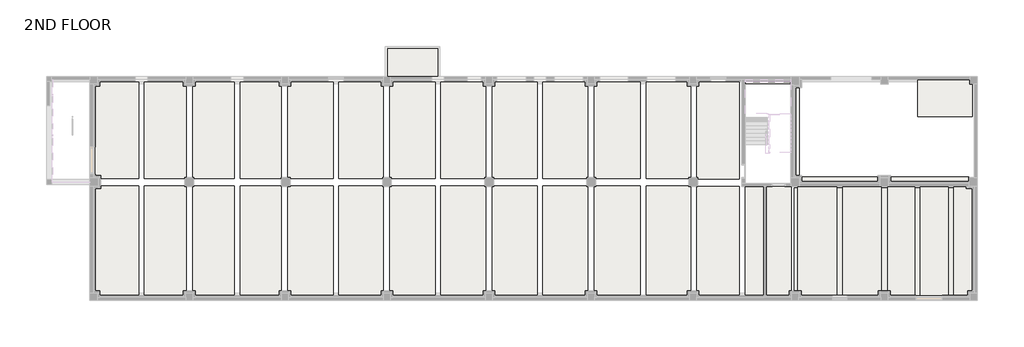
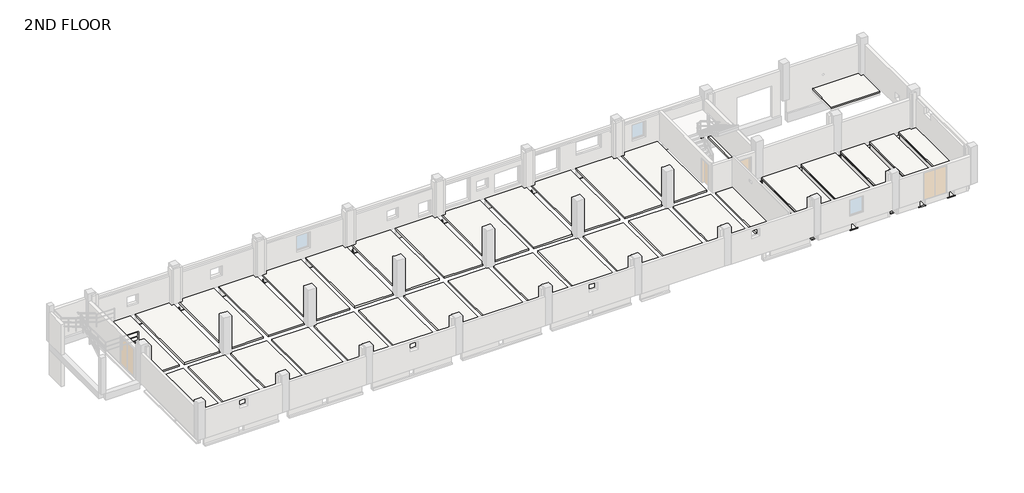
# One storey, part 4 of 7: 8 slabs, 2 coverings, 1 roof.
"""IFC4 building model written with IfcOpenShell, lengths in millimetres."""

from ifc_helpers import new_model, si_unit, frame, origin, place, context, project, spatial, polyline, outline, extrude, faceted_brep, element, save

model = new_model("IFC4")

# Units and contexts
model_context = context("Model", 3, world=origin())
ifc_project = project(units=[si_unit("LENGTHUNIT", "METRE", prefix="MILLI")], contexts=[model_context])

# Site, building, storey
site = spatial("IfcSite", under=ifc_project)
building = spatial("IfcBuilding", under=site)
storey = spatial("IfcBuildingStorey", under=building, Name="2ND FLOOR", Elevation=10600.0)

# Coverings
placement = place(None, origin())
element("IfcCovering", 1, ObjectType="H_CE_AR_B09_Souns Absorbing_100T_C7", at=placement, inside=storey, context=model_context, shape_type="SweptSolid", body=[
    extrude(outline(polyline([(58275.0, -8350.0), (58275.0, -16900.0), (55300.0, -16900.0), (55300.0, -16700.0), (55200.0, -16700.0), (55200.0, -8350.0), (58275.0, -8350.0)])), frame((0.0, 0.0, 10350.0), z_axis=(0.0, 0.0, 1.0), x_axis=(1.0, 0.0, 0.0)), (0.0, 0.0, 1.0), 100.0),
    extrude(outline(polyline([(58725.0, -8350.0), (61750.0, -8350.0), (61750.0, -16700.0), (61700.0, -16700.0), (61700.0, -16900.0), (58725.0, -16900.0), (58725.0, -8350.0)])), frame((0.0, 0.0, 10350.0), z_axis=(0.0, 0.0, 1.0), x_axis=(1.0, 0.0, 0.0)), (0.0, 0.0, 1.0), 100.0),
    extrude(outline(polyline([(64375.0, -8350.0), (64375.0, -16900.0), (62300.0, -16900.0), (62300.0, -16700.0), (62250.0, -16700.0), (62250.0, -8350.0), (64375.0, -8350.0)])), frame((0.0, 0.0, 10350.0), z_axis=(0.0, 0.0, 1.0), x_axis=(1.0, 0.0, 0.0)), (0.0, 0.0, 1.0), 100.0),
    extrude(outline(polyline([(67000.0, -8350.0), (67000.0, -16900.0), (64825.0, -16900.0), (64825.0, -8350.0), (67000.0, -8350.0)])), frame((0.0, 0.0, 10350.0), z_axis=(0.0, 0.0, 1.0), x_axis=(1.0, 0.0, 0.0)), (0.0, 0.0, 1.0), 100.0),
    extrude(outline(polyline([(68700.0, -16900.0), (67450.0, -16900.0), (67450.0, -8350.0), (68900.0, -8350.0), (68900.0, -16700.0), (68700.0, -16700.0), (68700.0, -16900.0)])), frame((0.0, 0.0, 10350.0), z_axis=(0.0, 0.0, 1.0), x_axis=(1.0, 0.0, 0.0)), (0.0, 0.0, 1.0), 100.0),
])
element("IfcCovering", 2, ObjectType="H_CE_AR_B09_Souns Absorbing_100T_C7", at=placement, inside=storey, context=model_context, shape_type="SweptSolid", body=[
    extrude(outline(polyline([(58175.0, -16886.0), (58175.0, -8469.0), (58825.0, -8469.0), (58825.0, -16886.0), (58175.0, -16886.0)])), frame((0.0, 0.0, 9700.0), z_axis=(0.0, 0.0, 1.0), x_axis=(1.0, 0.0, 0.0)), (0.0, 0.0, 1.0), 100.0),
    extrude(outline(polyline([(61650.0, -16536.0), (61650.0, -8469.0), (62350.0, -8469.0), (62350.0, -16536.0), (61650.0, -16536.0)])), frame((0.0, 0.0, 9700.0), z_axis=(0.0, 0.0, 1.0), x_axis=(1.0, 0.0, 0.0)), (0.0, 0.0, 1.0), 100.0),
    extrude(outline(polyline([(64275.0, -16886.0), (64275.0, -8469.0), (64925.0, -8469.0), (64925.0, -16886.0), (64275.0, -16886.0)])), frame((0.0, 0.0, 9700.0), z_axis=(0.0, 0.0, 1.0), x_axis=(1.0, 0.0, 0.0)), (0.0, 0.0, 1.0), 100.0),
    extrude(outline(polyline([(66900.0, -16886.0), (66900.0, -8469.0), (67550.0, -8469.0), (67550.0, -16886.0), (66900.0, -16886.0)])), frame((0.0, 0.0, 9700.0), z_axis=(0.0, 0.0, 1.0), x_axis=(1.0, 0.0, 0.0)), (0.0, 0.0, 1.0), 100.0),
    extrude(outline(polyline([(54937.0, -8469.0), (55300.0, -8469.0), (55300.0, -16536.0), (54937.0, -16536.0), (54937.0, -8469.0)])), frame((0.0, 0.0, 9700.0), z_axis=(0.0, 0.0, 1.0), x_axis=(1.0, 0.0, 0.0)), (0.0, 0.0, 1.0), 100.0),
])

# Roof
element("IfcRoof", 3, ObjectType="H_RF_AR_B06_RC Roof Finish_SkyPanel Roof_T160", at=placement, inside=storey, context=model_context, shape_type="SweptSolid", body=[
    extrude(outline(polyline([(23000.0, 2500.0), (27000.0, 2500.0), (27000.0, 300.0), (23000.0, 300.0), (23000.0, 2500.0)])), frame((0.0, 0.0, 9300.0), z_axis=(0.0, 0.0, 1.0), x_axis=(1.0, 0.0, 0.0)), (0.0, 0.0, 1.0), 170.0),
])

# Slabs
element("IfcSlab", 4, ObjectType="H_FL_AR_S17_RC Slab_T150_2S1", at=placement, inside=storey, context=model_context, shape_type="Brep", body=[
    faceted_brep([(3525.0, -100.0, 10450.0), (3525.0, -7700.0, 10450.0), (400.0, -7700.0, 10450.0), (399.4974747, -7700.0, 10450.0), (399.4974747, -7650.0, 10450.0), (100.0, -7650.0, 10450.0), (100.0, -300.0, 10450.0), (300.0, -300.0, 10450.0), (300.0, -100.0, 10450.0), (3525.0, -100.0, 10600.0), (300.0, -100.0, 10600.0), (300.0, -300.0, 10600.0), (100.0, -300.0, 10600.0), (100.0, -7650.0, 10600.0), (399.4974747, -7650.0, 10600.0), (399.4974747, -7700.0, 10600.0), (400.0, -7700.0, 10600.0), (3525.0, -7700.0, 10600.0)], [[[0, 1, 2, 3, 4, 5, 6, 7, 8]], [[9, 10, 11, 12, 13, 14, 15, 16, 17]], [[1, 0, 9, 17]], [[3, 2, 1, 17, 16, 15]], [[4, 3, 15, 14]], [[5, 4, 14, 13]], [[6, 5, 13, 12]], [[7, 6, 12, 11]], [[8, 7, 11, 10]], [[0, 8, 10, 9]]]),
    faceted_brep([(3975.0, -100.0, 10450.0), (7200.0, -100.0, 10450.0), (7200.0, -300.0, 10450.0), (7250.0, -300.0, 10450.0), (7250.0, -7650.0, 10450.0), (7150.0, -7650.0, 10450.0), (7150.0, -7700.0, 10450.0), (3975.0, -7700.0, 10450.0), (3975.0, -100.0, 10600.0), (3975.0, -7700.0, 10600.0), (7150.0, -7700.0, 10600.0), (7150.0, -7650.0, 10600.0), (7250.0, -7650.0, 10600.0), (7250.0, -300.0, 10600.0), (7200.0, -300.0, 10600.0), (7200.0, -100.0, 10600.0)], [[[0, 1, 2, 3, 4, 5, 6, 7]], [[8, 9, 10, 11, 12, 13, 14, 15]], [[1, 0, 8, 15]], [[2, 1, 15, 14]], [[3, 2, 14, 13]], [[4, 3, 13, 12]], [[5, 4, 12, 11]], [[6, 5, 11, 10]], [[7, 6, 10, 9]], [[0, 7, 9, 8]]]),
    faceted_brep([(3525.0, -16900.0, 10450.0), (300.0, -16900.0, 10450.0), (300.0, -16700.0, 10450.0), (100.0, -16700.0, 10450.0), (100.0, -8350.0, 10450.0), (399.4974747, -8350.0, 10450.0), (399.4974747, -8300.0, 10450.0), (400.0, -8300.0, 10450.0), (3525.0, -8300.0, 10450.0), (3525.0, -16900.0, 10600.0), (3525.0, -8300.0, 10600.0), (400.0, -8300.0, 10600.0), (399.4974747, -8300.0, 10600.0), (399.4974747, -8350.0, 10600.0), (100.0, -8350.0, 10600.0), (100.0, -16700.0, 10600.0), (300.0, -16700.0, 10600.0), (300.0, -16900.0, 10600.0)], [[[0, 1, 2, 3, 4, 5, 6, 7, 8]], [[9, 10, 11, 12, 13, 14, 15, 16, 17]], [[1, 0, 9, 17]], [[2, 1, 17, 16]], [[3, 2, 16, 15]], [[4, 3, 15, 14]], [[5, 4, 14, 13]], [[6, 5, 13, 12]], [[8, 7, 6, 12, 11, 10]], [[0, 8, 10, 9]]]),
    faceted_brep([(3975.0, -16900.0, 10450.0), (3975.0, -8300.0, 10450.0), (7150.0, -8300.0, 10450.0), (7150.0, -8350.0, 10450.0), (7250.0, -8350.0, 10450.0), (7250.0, -16700.0, 10450.0), (7200.0, -16700.0, 10450.0), (7200.0, -16900.0, 10450.0), (3975.0, -16900.0, 10600.0), (7200.0, -16900.0, 10600.0), (7200.0, -16700.0, 10600.0), (7250.0, -16700.0, 10600.0), (7250.0, -8350.0, 10600.0), (7150.0, -8350.0, 10600.0), (7150.0, -8300.0, 10600.0), (3975.0, -8300.0, 10600.0)], [[[0, 1, 2, 3, 4, 5, 6, 7]], [[8, 9, 10, 11, 12, 13, 14, 15]], [[1, 0, 8, 15]], [[2, 1, 15, 14]], [[3, 2, 14, 13]], [[4, 3, 13, 12]], [[5, 4, 12, 11]], [[6, 5, 11, 10]], [[7, 6, 10, 9]], [[0, 7, 9, 8]]]),
    faceted_brep([(11025.0, -100.0, 10450.0), (11025.0, -7700.0, 10450.0), (7850.0, -7700.0, 10450.0), (7850.0, -7650.0, 10450.0), (7750.0, -7650.0, 10450.0), (7750.0, -300.0, 10450.0), (7800.0, -300.0, 10450.0), (7800.0, -100.0, 10450.0), (11025.0, -100.0, 10600.0), (7800.0, -100.0, 10600.0), (7800.0, -300.0, 10600.0), (7750.0, -300.0, 10600.0), (7750.0, -7650.0, 10600.0), (7850.0, -7650.0, 10600.0), (7850.0, -7700.0, 10600.0), (11025.0, -7700.0, 10600.0)], [[[0, 1, 2, 3, 4, 5, 6, 7]], [[8, 9, 10, 11, 12, 13, 14, 15]], [[1, 0, 8, 15]], [[2, 1, 15, 14]], [[3, 2, 14, 13]], [[4, 3, 13, 12]], [[5, 4, 12, 11]], [[6, 5, 11, 10]], [[7, 6, 10, 9]], [[0, 7, 9, 8]]]),
    faceted_brep([(11025.0, -16900.0, 10450.0), (7800.0, -16900.0, 10450.0), (7800.0, -16700.0, 10450.0), (7750.0, -16700.0, 10450.0), (7750.0, -8350.0, 10450.0), (7850.0, -8350.0, 10450.0), (7850.0, -8300.0, 10450.0), (11025.0, -8300.0, 10450.0), (11025.0, -16900.0, 10600.0), (11025.0, -8300.0, 10600.0), (7850.0, -8300.0, 10600.0), (7850.0, -8350.0, 10600.0), (7750.0, -8350.0, 10600.0), (7750.0, -16700.0, 10600.0), (7800.0, -16700.0, 10600.0), (7800.0, -16900.0, 10600.0)], [[[0, 1, 2, 3, 4, 5, 6, 7]], [[8, 9, 10, 11, 12, 13, 14, 15]], [[1, 0, 8, 15]], [[2, 1, 15, 14]], [[3, 2, 14, 13]], [[4, 3, 13, 12]], [[5, 4, 12, 11]], [[6, 5, 11, 10]], [[7, 6, 10, 9]], [[0, 7, 9, 8]]]),
    faceted_brep([(14700.0, -100.0, 10450.0), (14700.0, -7700.0, 10450.0), (11475.0, -7700.0, 10450.0), (11475.0, -100.0, 10450.0), (14700.0, -100.0, 10600.0), (11475.0, -100.0, 10600.0), (11475.0, -7700.0, 10600.0), (14700.0, -7700.0, 10600.0), (14700.0, -7650.0, 10600.0), (14700.0, -300.0, 10600.0)], [[[0, 1, 2, 3]], [[4, 5, 6, 7, 8, 9]], [[1, 0, 4, 9, 8, 7]], [[2, 1, 7, 6]], [[3, 2, 6, 5]], [[0, 3, 5, 4]]]),
    faceted_brep([(11475.0, -8300.0, 10450.0), (14700.0, -8300.0, 10450.0), (14700.0, -16900.0, 10450.0), (11475.0, -16900.0, 10450.0), (11475.0, -8300.0, 10600.0), (11475.0, -16900.0, 10600.0), (14700.0, -16900.0, 10600.0), (14700.0, -16700.0, 10600.0), (14700.0, -8350.0, 10600.0), (14700.0, -8300.0, 10600.0)], [[[0, 1, 2, 3]], [[4, 5, 6, 7, 8, 9]], [[1, 0, 4, 9]], [[2, 1, 9, 8, 7, 6]], [[3, 2, 6, 5]], [[0, 3, 5, 4]]]),
    faceted_brep([(15300.0, -300.0, 10450.0), (15300.0, -100.0, 10450.0), (18775.0, -100.0, 10450.0), (18775.0, -7700.0, 10450.0), (15400.0000001, -7700.0, 10450.0), (15400.0000001, -7650.0, 10450.0), (15200.0, -7650.0, 10450.0), (15200.0, -300.0, 10450.0), (15300.0, -300.0, 10600.0), (15200.0, -300.0, 10600.0), (15200.0, -7650.0, 10600.0), (15400.0000001, -7650.0, 10600.0), (15400.0000001, -7700.0, 10600.0), (18775.0, -7700.0, 10600.0), (18775.0, -100.0, 10600.0), (15300.0, -100.0, 10600.0)], [[[0, 1, 2, 3, 4, 5, 6, 7]], [[8, 9, 10, 11, 12, 13, 14, 15]], [[1, 0, 8, 15]], [[2, 1, 15, 14]], [[3, 2, 14, 13]], [[4, 3, 13, 12]], [[5, 4, 12, 11]], [[6, 5, 11, 10]], [[7, 6, 10, 9]], [[0, 7, 9, 8]]]),
    faceted_brep([(15300.0, -16700.0, 10450.0), (15200.0, -16700.0, 10450.0), (15200.0, -8350.0, 10450.0), (15400.0000001, -8350.0, 10450.0), (15400.0000001, -8300.0, 10450.0), (18775.0, -8300.0, 10450.0), (18775.0, -16900.0, 10450.0), (15300.0, -16900.0, 10450.0), (15300.0, -16700.0, 10600.0), (15300.0, -16900.0, 10600.0), (18775.0, -16900.0, 10600.0), (18775.0, -8300.0, 10600.0), (15400.0000001, -8300.0, 10600.0), (15400.0000001, -8350.0, 10600.0), (15200.0, -8350.0, 10600.0), (15200.0, -16700.0, 10600.0)], [[[0, 1, 2, 3, 4, 5, 6, 7]], [[8, 9, 10, 11, 12, 13, 14, 15]], [[1, 0, 8, 15]], [[2, 1, 15, 14]], [[3, 2, 14, 13]], [[4, 3, 13, 12]], [[5, 4, 12, 11]], [[6, 5, 11, 10]], [[7, 6, 10, 9]], [[0, 7, 9, 8]]]),
    faceted_brep([(19225.0, -100.0, 10450.0), (22700.0, -100.0, 10450.0), (22700.0, -7650.0, 10450.0), (22650.0000003, -7650.0, 10450.0), (22650.0000003, -7700.0, 10450.0), (19225.0, -7700.0, 10450.0), (19225.0, -100.0, 10600.0), (19225.0, -7700.0, 10600.0), (22650.0000003, -7700.0, 10600.0), (22650.0000003, -7650.0, 10600.0), (22700.0, -7650.0, 10600.0), (22700.0, -300.0, 10600.0), (22700.0, -100.0, 10600.0)], [[[0, 1, 2, 3, 4, 5]], [[6, 7, 8, 9, 10, 11, 12]], [[1, 0, 6, 12]], [[2, 1, 12, 11, 10]], [[3, 2, 10, 9]], [[4, 3, 9, 8]], [[5, 4, 8, 7]], [[0, 5, 7, 6]]]),
    faceted_brep([(19225.0, -16900.0, 10450.0), (19225.0, -8300.0, 10450.0), (22650.0000003, -8300.0, 10450.0), (22650.0000003, -8350.0, 10450.0), (22700.0, -8350.0, 10450.0), (22700.0, -16900.0, 10450.0), (19225.0, -16900.0, 10600.0), (22700.0, -16900.0, 10600.0), (22700.0, -16700.0, 10600.0), (22700.0, -8350.0, 10600.0), (22650.0000003, -8350.0, 10600.0), (22650.0000003, -8300.0, 10600.0), (19225.0, -8300.0, 10600.0)], [[[0, 1, 2, 3, 4, 5]], [[6, 7, 8, 9, 10, 11, 12]], [[1, 0, 6, 12]], [[2, 1, 12, 11]], [[3, 2, 11, 10]], [[4, 3, 10, 9]], [[5, 4, 9, 8, 7]], [[0, 5, 7, 6]]]),
    faceted_brep([(23300.0, -100.0, 10450.0), (26775.0, -100.0, 10450.0), (26775.0, -7700.0, 10450.0), (23350.0000003, -7700.0, 10450.0), (23350.0000003, -7650.0, 10450.0), (23200.0, -7650.0, 10450.0), (23200.0, -300.0, 10450.0), (23300.0, -300.0, 10450.0), (23300.0, -100.0, 10600.0), (23300.0, -300.0, 10600.0), (23200.0, -300.0, 10600.0), (23200.0, -7650.0, 10600.0), (23350.0000003, -7650.0, 10600.0), (23350.0000003, -7700.0, 10600.0), (26775.0, -7700.0, 10600.0), (26775.0, -100.0, 10600.0)], [[[0, 1, 2, 3, 4, 5, 6, 7]], [[8, 9, 10, 11, 12, 13, 14, 15]], [[1, 0, 8, 15]], [[2, 1, 15, 14]], [[3, 2, 14, 13]], [[4, 3, 13, 12]], [[5, 4, 12, 11]], [[6, 5, 11, 10]], [[7, 6, 10, 9]], [[0, 7, 9, 8]]]),
    faceted_brep([(23300.0, -16900.0, 10450.0), (23300.0, -16700.0, 10450.0), (23200.0, -16700.0, 10450.0), (23200.0, -8350.0, 10450.0), (23350.0000003, -8350.0, 10450.0), (23350.0000003, -8300.0, 10450.0), (26775.0, -8300.0, 10450.0), (26775.0, -16900.0, 10450.0), (23300.0, -16900.0, 10600.0), (26775.0, -16900.0, 10600.0), (26775.0, -8300.0, 10600.0), (23350.0000003, -8300.0, 10600.0), (23350.0000003, -8350.0, 10600.0), (23200.0, -8350.0, 10600.0), (23200.0, -16700.0, 10600.0), (23300.0, -16700.0, 10600.0)], [[[0, 1, 2, 3, 4, 5, 6, 7]], [[8, 9, 10, 11, 12, 13, 14, 15]], [[1, 0, 8, 15]], [[2, 1, 15, 14]], [[3, 2, 14, 13]], [[4, 3, 13, 12]], [[5, 4, 12, 11]], [[6, 5, 11, 10]], [[7, 6, 10, 9]], [[0, 7, 9, 8]]]),
    faceted_brep([(30700.0, -100.0, 10450.0), (30700.0, -300.0, 10450.0), (30750.0000002, -300.0, 10450.0), (30750.0000002, -7650.0, 10450.0), (30649.9999997, -7650.0, 10450.0), (30649.9999997, -7700.0, 10450.0), (27225.0, -7700.0, 10450.0), (27225.0, -100.0, 10450.0), (30700.0, -100.0, 10600.0), (27225.0, -100.0, 10600.0), (27225.0, -7700.0, 10600.0), (30649.9999997, -7700.0, 10600.0), (30649.9999997, -7650.0, 10600.0), (30750.0000002, -7650.0, 10600.0), (30750.0000002, -300.0, 10600.0), (30700.0, -300.0, 10600.0)], [[[0, 1, 2, 3, 4, 5, 6, 7]], [[8, 9, 10, 11, 12, 13, 14, 15]], [[1, 0, 8, 15]], [[2, 1, 15, 14]], [[3, 2, 14, 13]], [[4, 3, 13, 12]], [[5, 4, 12, 11]], [[6, 5, 11, 10]], [[7, 6, 10, 9]], [[0, 7, 9, 8]]]),
    faceted_brep([(30700.0, -16900.0, 10450.0), (27225.0, -16900.0, 10450.0), (27225.0, -8300.0, 10450.0), (30649.9999997, -8300.0, 10450.0), (30649.9999997, -8350.0, 10450.0), (30750.0000002, -8350.0, 10450.0), (30750.0000002, -16700.0, 10450.0), (30700.0, -16700.0, 10450.0), (30700.0, -16900.0, 10600.0), (30700.0, -16700.0, 10600.0), (30750.0000002, -16700.0, 10600.0), (30750.0000002, -8350.0, 10600.0), (30649.9999997, -8350.0, 10600.0), (30649.9999997, -8300.0, 10600.0), (27225.0, -8300.0, 10600.0), (27225.0, -16900.0, 10600.0)], [[[0, 1, 2, 3, 4, 5, 6, 7]], [[8, 9, 10, 11, 12, 13, 14, 15]], [[1, 0, 8, 15]], [[2, 1, 15, 14]], [[3, 2, 14, 13]], [[4, 3, 13, 12]], [[5, 4, 12, 11]], [[6, 5, 11, 10]], [[7, 6, 10, 9]], [[0, 7, 9, 8]]]),
    faceted_brep([(31300.0, -100.0, 10450.0), (34775.0, -100.0, 10450.0), (34775.0, -7700.0, 10450.0), (31350.0000003, -7700.0, 10450.0), (31350.0000003, -7650.0, 10450.0), (31249.9999998, -7650.0, 10450.0), (31249.9999998, -300.0, 10450.0), (31300.0, -300.0, 10450.0), (31300.0, -100.0, 10600.0), (31300.0, -300.0, 10600.0), (31249.9999998, -300.0, 10600.0), (31249.9999998, -7650.0, 10600.0), (31350.0000003, -7650.0, 10600.0), (31350.0000003, -7700.0, 10600.0), (34775.0, -7700.0, 10600.0), (34775.0, -100.0, 10600.0)], [[[0, 1, 2, 3, 4, 5, 6, 7]], [[8, 9, 10, 11, 12, 13, 14, 15]], [[1, 0, 8, 15]], [[2, 1, 15, 14]], [[3, 2, 14, 13]], [[4, 3, 13, 12]], [[5, 4, 12, 11]], [[6, 5, 11, 10]], [[7, 6, 10, 9]], [[0, 7, 9, 8]]]),
    faceted_brep([(31300.0, -16900.0, 10450.0), (31300.0, -16700.0, 10450.0), (31249.9999998, -16700.0, 10450.0), (31249.9999998, -8350.0, 10450.0), (31350.0000003, -8350.0, 10450.0), (31350.0000003, -8300.0, 10450.0), (34775.0, -8300.0, 10450.0), (34775.0, -16900.0, 10450.0), (31300.0, -16900.0, 10600.0), (34775.0, -16900.0, 10600.0), (34775.0, -8300.0, 10600.0), (31350.0000003, -8300.0, 10600.0), (31350.0000003, -8350.0, 10600.0), (31249.9999998, -8350.0, 10600.0), (31249.9999998, -16700.0, 10600.0), (31300.0, -16700.0, 10600.0)], [[[0, 1, 2, 3, 4, 5, 6, 7]], [[8, 9, 10, 11, 12, 13, 14, 15]], [[1, 0, 8, 15]], [[2, 1, 15, 14]], [[3, 2, 14, 13]], [[4, 3, 13, 12]], [[5, 4, 12, 11]], [[6, 5, 11, 10]], [[7, 6, 10, 9]], [[0, 7, 9, 8]]]),
    faceted_brep([(38700.0, -100.0, 10450.0), (38700.0, -300.0, 10450.0), (38750.0000002, -300.0, 10450.0), (38750.0000002, -7650.0, 10450.0), (38649.9999997, -7650.0, 10450.0), (38649.9999997, -7700.0, 10450.0), (35225.0, -7700.0, 10450.0), (35225.0, -100.0, 10450.0), (38700.0, -100.0, 10600.0), (35225.0, -100.0, 10600.0), (35225.0, -7700.0, 10600.0), (38649.9999997, -7700.0, 10600.0), (38649.9999997, -7650.0, 10600.0), (38750.0000002, -7650.0, 10600.0), (38750.0000002, -300.0, 10600.0), (38700.0, -300.0, 10600.0)], [[[0, 1, 2, 3, 4, 5, 6, 7]], [[8, 9, 10, 11, 12, 13, 14, 15]], [[1, 0, 8, 15]], [[2, 1, 15, 14]], [[3, 2, 14, 13]], [[4, 3, 13, 12]], [[5, 4, 12, 11]], [[6, 5, 11, 10]], [[7, 6, 10, 9]], [[0, 7, 9, 8]]]),
    faceted_brep([(38700.0, -16900.0, 10450.0), (35225.0, -16900.0, 10450.0), (35225.0, -8300.0, 10450.0), (38649.9999997, -8300.0, 10450.0), (38649.9999997, -8350.0, 10450.0), (38750.0000002, -8350.0, 10450.0), (38750.0000002, -16700.0, 10450.0), (38700.0, -16700.0, 10450.0), (38700.0, -16900.0, 10600.0), (38700.0, -16700.0, 10600.0), (38750.0000002, -16700.0, 10600.0), (38750.0000002, -8350.0, 10600.0), (38649.9999997, -8350.0, 10600.0), (38649.9999997, -8300.0, 10600.0), (35225.0, -8300.0, 10600.0), (35225.0, -16900.0, 10600.0)], [[[0, 1, 2, 3, 4, 5, 6, 7]], [[8, 9, 10, 11, 12, 13, 14, 15]], [[1, 0, 8, 15]], [[2, 1, 15, 14]], [[3, 2, 14, 13]], [[4, 3, 13, 12]], [[5, 4, 12, 11]], [[6, 5, 11, 10]], [[7, 6, 10, 9]], [[0, 7, 9, 8]]]),
    faceted_brep([(39300.0, -100.0, 10450.0), (42875.0, -100.0, 10450.0), (42875.0, -7700.0, 10450.0), (39350.0000003, -7700.0, 10450.0), (39350.0000003, -7650.0, 10450.0), (39249.9999998, -7650.0, 10450.0), (39249.9999998, -300.0, 10450.0), (39300.0, -300.0, 10450.0), (39300.0, -100.0, 10600.0), (39300.0, -300.0, 10600.0), (39249.9999998, -300.0, 10600.0), (39249.9999998, -7650.0, 10600.0), (39350.0000003, -7650.0, 10600.0), (39350.0000003, -7700.0, 10600.0), (42875.0, -7700.0, 10600.0), (42875.0, -100.0, 10600.0)], [[[0, 1, 2, 3, 4, 5, 6, 7]], [[8, 9, 10, 11, 12, 13, 14, 15]], [[1, 0, 8, 15]], [[2, 1, 15, 14]], [[3, 2, 14, 13]], [[4, 3, 13, 12]], [[5, 4, 12, 11]], [[6, 5, 11, 10]], [[7, 6, 10, 9]], [[0, 7, 9, 8]]]),
    faceted_brep([(39300.0, -16900.0, 10450.0), (39300.0, -16700.0, 10450.0), (39249.9999998, -16700.0, 10450.0), (39249.9999998, -8350.0, 10450.0), (39350.0000003, -8350.0, 10450.0), (39350.0000003, -8300.0, 10450.0), (42875.0, -8300.0, 10450.0), (42875.0, -16900.0, 10450.0), (39300.0, -16900.0, 10600.0), (42875.0, -16900.0, 10600.0), (42875.0, -8300.0, 10600.0), (39350.0000003, -8300.0, 10600.0), (39350.0000003, -8350.0, 10600.0), (39249.9999998, -8350.0, 10600.0), (39249.9999998, -16700.0, 10600.0), (39300.0, -16700.0, 10600.0)], [[[0, 1, 2, 3, 4, 5, 6, 7]], [[8, 9, 10, 11, 12, 13, 14, 15]], [[1, 0, 8, 15]], [[2, 1, 15, 14]], [[3, 2, 14, 13]], [[4, 3, 13, 12]], [[5, 4, 12, 11]], [[6, 5, 11, 10]], [[7, 6, 10, 9]], [[0, 7, 9, 8]]]),
    faceted_brep([(46700.0, -100.0, 10450.0), (46700.0, -300.0, 10450.0), (46800.0, -300.0, 10450.0), (46800.0, -7650.0, 10450.0), (46649.9999999, -7650.0, 10450.0), (46649.9999999, -7700.0, 10450.0), (43325.0, -7700.0, 10450.0), (43325.0, -100.0, 10450.0), (46700.0, -100.0, 10600.0), (43325.0, -100.0, 10600.0), (43325.0, -7700.0, 10600.0), (46649.9999999, -7700.0, 10600.0), (46649.9999999, -7650.0, 10600.0), (46800.0, -7650.0, 10600.0), (46800.0, -300.0, 10600.0), (46700.0, -300.0, 10600.0)], [[[0, 1, 2, 3, 4, 5, 6, 7]], [[8, 9, 10, 11, 12, 13, 14, 15]], [[1, 0, 8, 15]], [[2, 1, 15, 14]], [[3, 2, 14, 13]], [[4, 3, 13, 12]], [[5, 4, 12, 11]], [[6, 5, 11, 10]], [[7, 6, 10, 9]], [[0, 7, 9, 8]]]),
    faceted_brep([(46700.0, -16900.0, 10450.0), (43325.0, -16900.0, 10450.0), (43325.0, -8300.0, 10450.0), (46649.9999999, -8300.0, 10450.0), (46649.9999999, -8350.0, 10450.0), (46800.0, -8350.0, 10450.0), (46800.0, -16700.0, 10450.0), (46700.0, -16700.0, 10450.0), (46700.0, -16900.0, 10600.0), (46700.0, -16700.0, 10600.0), (46800.0, -16700.0, 10600.0), (46800.0, -8350.0, 10600.0), (46649.9999999, -8350.0, 10600.0), (46649.9999999, -8300.0, 10600.0), (43325.0, -8300.0, 10600.0), (43325.0, -16900.0, 10600.0)], [[[0, 1, 2, 3, 4, 5, 6, 7]], [[8, 9, 10, 11, 12, 13, 14, 15]], [[1, 0, 8, 15]], [[2, 1, 15, 14]], [[3, 2, 14, 13]], [[4, 3, 13, 12]], [[5, 4, 12, 11]], [[6, 5, 11, 10]], [[7, 6, 10, 9]], [[0, 7, 9, 8]]]),
    faceted_brep([(50625.0, -8350.0, 10450.0), (50625.0, -16900.0, 10450.0), (47300.0, -16900.0, 10450.0), (47300.0, -8350.0, 10450.0), (50625.0, -8350.0, 10600.0), (47350.0, -8350.0, 10600.0), (47300.0, -8350.0, 10600.0), (47300.0, -16700.0, 10600.0), (47300.0, -16900.0, 10600.0), (50625.0, -16900.0, 10600.0)], [[[0, 1, 2, 3]], [[4, 5, 6, 7, 8, 9]], [[1, 0, 4, 9]], [[2, 1, 9, 8]], [[3, 2, 8, 7, 6]], [[0, 3, 6, 5, 4]]]),
    faceted_brep([(50625.0, -100.0, 10450.0), (50625.0, -7750.0, 10450.0), (47349.9999999, -7750.0, 10450.0), (47349.9999999, -7650.0, 10450.0), (47300.0, -7650.0, 10450.0), (47300.0, -100.0, 10450.0), (50625.0, -100.0, 10600.0), (47300.0, -100.0, 10600.0), (47300.0, -300.0, 10600.0), (47300.0, -7650.0, 10600.0), (47349.9999999, -7650.0, 10600.0), (47349.9999999, -7750.0, 10600.0), (50625.0, -7750.0, 10600.0)], [[[0, 1, 2, 3, 4, 5]], [[6, 7, 8, 9, 10, 11, 12]], [[1, 0, 6, 12]], [[2, 1, 12, 11]], [[3, 2, 11, 10]], [[4, 3, 10, 9]], [[5, 4, 9, 8, 7]], [[0, 5, 7, 6]]]),
    faceted_brep([(54700.0, -8350.0, 10450.0), (54700.0, -16900.0, 10450.0), (51075.0, -16900.0, 10450.0), (51075.0, -8350.0, 10450.0), (54700.0, -8350.0, 10600.0), (54650.0, -8350.0, 10600.0), (51075.0, -8350.0, 10600.0), (51075.0, -16900.0, 10600.0), (54700.0, -16900.0, 10600.0), (54700.0, -16700.0, 10600.0)], [[[0, 1, 2, 3]], [[4, 5, 6, 7, 8, 9]], [[1, 0, 4, 9, 8]], [[2, 1, 8, 7]], [[3, 2, 7, 6]], [[0, 3, 6, 5, 4]]]),
    faceted_brep([(58275.0, -8350.0, 10450.0), (58275.0, -16900.0, 10450.0), (55300.0, -16900.0, 10450.0), (55300.0, -16700.0, 10450.0), (55200.0, -16700.0, 10450.0), (55200.0, -8350.0, 10450.0), (58275.0, -8350.0, 10600.0), (55350.0, -8350.0, 10600.0), (55200.0, -8350.0, 10600.0), (55200.0, -16700.0, 10600.0), (55300.0, -16700.0, 10600.0), (55300.0, -16900.0, 10600.0), (58275.0, -16900.0, 10600.0)], [[[0, 1, 2, 3, 4, 5]], [[6, 7, 8, 9, 10, 11, 12]], [[1, 0, 6, 12]], [[2, 1, 12, 11]], [[3, 2, 11, 10]], [[4, 3, 10, 9]], [[5, 4, 9, 8]], [[0, 5, 8, 7, 6]]]),
    faceted_brep([(58725.0, -8350.0, 10450.0), (61750.0, -8350.0, 10450.0), (61750.0, -16700.0, 10450.0), (61700.0, -16700.0, 10450.0), (61700.0, -16900.0, 10450.0), (58725.0, -16900.0, 10450.0), (58725.0, -8350.0, 10600.0), (58725.0, -16900.0, 10600.0), (61700.0, -16900.0, 10600.0), (61700.0, -16700.0, 10600.0), (61750.0, -16700.0, 10600.0), (61750.0, -8350.0, 10600.0), (61650.0, -8350.0, 10600.0)], [[[0, 1, 2, 3, 4, 5]], [[6, 7, 8, 9, 10, 11, 12]], [[1, 0, 6, 12, 11]], [[2, 1, 11, 10]], [[3, 2, 10, 9]], [[4, 3, 9, 8]], [[5, 4, 8, 7]], [[0, 5, 7, 6]]]),
    faceted_brep([(64375.0, -8350.0, 10450.0), (64375.0, -16900.0, 10450.0), (62300.0, -16900.0, 10450.0), (62300.0, -16700.0, 10450.0), (62250.0, -16700.0, 10450.0), (62250.0, -8350.0, 10450.0), (64375.0, -8350.0, 10600.0), (62350.0, -8350.0, 10600.0), (62250.0, -8350.0, 10600.0), (62250.0, -16700.0, 10600.0), (62300.0, -16700.0, 10600.0), (62300.0, -16900.0, 10600.0), (64375.0, -16900.0, 10600.0)], [[[0, 1, 2, 3, 4, 5]], [[6, 7, 8, 9, 10, 11, 12]], [[1, 0, 6, 12]], [[2, 1, 12, 11]], [[3, 2, 11, 10]], [[4, 3, 10, 9]], [[5, 4, 9, 8]], [[0, 5, 8, 7, 6]]]),
    faceted_brep([(67000.0, -8350.0, 10450.0), (67000.0, -16900.0, 10450.0), (64825.0, -16900.0, 10450.0), (64825.0, -8350.0, 10450.0), (67000.0, -8350.0, 10600.0), (64825.0, -8350.0, 10600.0), (64825.0, -16900.0, 10600.0), (67000.0, -16900.0, 10600.0)], [[[0, 1, 2, 3]], [[4, 5, 6, 7]], [[1, 0, 4, 7]], [[2, 1, 7, 6]], [[3, 2, 6, 5]], [[0, 3, 5, 4]]]),
    faceted_brep([(68700.0, -16900.0, 10450.0), (67450.0, -16900.0, 10450.0), (67450.0, -8350.0, 10450.0), (68900.0, -8350.0, 10450.0), (68900.0, -16700.0, 10450.0), (68700.0, -16700.0, 10450.0), (68700.0, -16900.0, 10600.0), (68700.0, -16700.0, 10600.0), (68900.0, -16700.0, 10600.0), (68900.0, -8350.0, 10600.0), (68600.0, -8350.0, 10600.0), (67450.0, -8350.0, 10600.0), (67450.0, -16900.0, 10600.0)], [[[0, 1, 2, 3, 4, 5]], [[6, 7, 8, 9, 10, 11, 12]], [[1, 0, 6, 12]], [[2, 1, 12, 11]], [[3, 2, 11, 10, 9]], [[4, 3, 9, 8]], [[5, 4, 8, 7]], [[0, 5, 7, 6]]]),
])
element("IfcSlab", 5, ObjectType="H_FL_AR_S17_RC Slab_T150_2S2", at=placement, inside=storey, context=model_context, shape_type="SweptSolid", body=[
    extrude(outline(polyline([(68900.0, -2850.0), (64600.0, -2850.0), (64600.0, 50.0), (68700.0, 50.0), (68700.0, -300.0), (68900.0, -300.0), (68900.0, -2850.0)])), frame((0.0, 0.0, 10450.0), z_axis=(0.0, 0.0, 1.0), x_axis=(1.0, 0.0, 0.0)), (0.0, 0.0, 1.0), 150.0),
])
element("IfcSlab", 6, ObjectType="H_FL_AR_S17_RC Slab_T150_2CS1", at=placement, inside=storey, context=model_context, shape_type="SweptSolid", body=[
    extrude(outline(polyline([(26850.0, 2350.0), (26850.0, 300.0), (23150.0, 300.0), (23150.0, 2350.0), (26850.0, 2350.0)])), frame((0.0, 0.0, 9150.0), z_axis=(0.0, 0.0, 1.0), x_axis=(1.0, 0.0, 0.0)), (0.0, 0.0, 1.0), 150.0),
])
element("IfcSlab", 7, ObjectType="H_FL_AR_B07l_2L Gypsum_Insulationl_T154", at=placement, inside=storey, context=model_context, shape_type="Brep", body=[
    faceted_brep([(54910.0, -7486.0, 10600.0), (54910.0, -564.0, 10600.0), (55160.0, -564.0, 10600.0), (55160.0, -7486.0, 10600.0), (55314.0, -564.0, 10754.0), (55064.0, -564.0, 10754.0), (54910.0, -564.0, 10754.0), (54910.0, -7486.0, 10754.0), (55064.0, -7486.0, 10754.0), (55314.0, -7486.0, 10754.0), (55314.0, -564.0, 10735.0), (55160.0, -564.0, 10735.0), (55314.0, -7486.0, 10735.0), (54910.0, -7486.0, 10735.0), (55160.0, -7486.0, 10735.0)], [[[0, 1, 2, 3]], [[4, 5, 6, 7, 8, 9]], [[6, 5, 4, 10, 11, 2, 1]], [[4, 9, 12, 10]], [[9, 8, 7, 13, 0, 3, 14, 12]], [[1, 0, 13, 7, 6]], [[11, 14, 3, 2]], [[14, 11, 10, 12]]]),
    faceted_brep([(61486.0, -8090.0, 10600.0), (55514.0, -8090.0, 10600.0), (55514.0, -7740.0, 10600.0), (61486.0, -7740.0, 10600.0), (61486.0, -8090.0, 10754.0), (61486.0, -7936.0, 10754.0), (61486.0, -7586.0, 10754.0), (55514.0, -7586.0, 10754.0), (55514.0, -7936.0, 10754.0), (55514.0, -8090.0, 10754.0), (61486.0, -8090.0, 10735.0), (61486.0, -7740.0, 10735.0), (61486.0, -7586.0, 10735.0), (55514.0, -8090.0, 10735.0), (55514.0, -7586.0, 10735.0), (55514.0, -7740.0, 10735.0)], [[[0, 1, 2, 3]], [[4, 5, 6, 7, 8, 9]], [[6, 5, 4, 10, 0, 3, 11, 12]], [[1, 0, 10, 4, 9, 13]], [[9, 8, 7, 14, 15, 2, 1, 13]], [[7, 6, 12, 14]], [[15, 11, 3, 2]], [[11, 15, 14, 12]]]),
    faceted_brep([(68600.0, -8090.0, 10600.0), (62514.0, -8090.0, 10600.0), (62514.0, -7740.0, 10600.0), (68600.0, -7740.0, 10600.0), (68600.0, -8090.0, 10754.0), (68600.0, -7936.0, 10754.0), (68600.0, -7586.0, 10754.0), (62514.0, -7586.0, 10754.0), (62514.0, -7936.0, 10754.0), (62514.0, -8090.0, 10754.0), (68600.0, -7740.0, 10735.0), (68600.0, -7586.0, 10735.0), (62514.0, -7586.0, 10735.0), (62514.0, -7740.0, 10735.0)], [[[0, 1, 2, 3]], [[4, 5, 6, 7, 8, 9]], [[6, 5, 4, 0, 3, 10, 11]], [[1, 0, 4, 9]], [[9, 8, 7, 12, 13, 2, 1]], [[7, 6, 11, 12]], [[13, 10, 3, 2]], [[10, 13, 12, 11]]]),
])
element("IfcSlab", 8, ObjectType="H_WA_AR_B02_Int Wall_2L Gypsum_Insulationl_T154(Mirror)", at=placement, inside=storey, context=model_context, shape_type="Brep", body=[
    faceted_brep([(54910.0, -564.0, 9646.0), (55064.0, -564.0, 9646.0), (55314.0, -564.0, 9646.0), (55314.0, -7486.0, 9646.0), (55064.0, -7486.0, 9646.0), (54910.0, -7486.0, 9646.0), (54910.0, -564.0, 9800.0), (54910.0, -7486.0, 9800.0), (55160.0, -7486.0, 9800.0), (55160.0, -564.0, 9800.0), (55160.0, -564.0, 9665.0), (55314.0, -564.0, 9665.0), (55314.0, -7486.0, 9665.0), (55160.0, -7486.0, 9665.0), (54910.0, -7486.0, 9665.0)], [[[0, 1, 2, 3, 4, 5]], [[6, 7, 8, 9]], [[2, 1, 0, 6, 9, 10, 11]], [[3, 2, 11, 12]], [[5, 4, 3, 12, 13, 8, 7, 14]], [[0, 5, 14, 7, 6]], [[13, 10, 9, 8]], [[10, 13, 12, 11]]]),
    faceted_brep([(61486.0, -7586.0, 9646.0), (61486.0, -7936.0, 9646.0), (61486.0, -8090.0, 9646.0), (55514.0, -8090.0, 9646.0), (55514.0, -7936.0, 9646.0), (55514.0, -7586.0, 9646.0), (55514.0, -8090.0, 9800.0), (61486.0, -8090.0, 9800.0), (61486.0, -7740.0, 9800.0), (55514.0, -7740.0, 9800.0), (61486.0, -7586.0, 9665.0), (61486.0, -7740.0, 9665.0), (61486.0, -8090.0, 9665.0), (55514.0, -8090.0, 9665.0), (55514.0, -7740.0, 9665.0), (55514.0, -7586.0, 9665.0)], [[[0, 1, 2, 3, 4, 5]], [[6, 7, 8, 9]], [[2, 1, 0, 10, 11, 8, 7, 12]], [[3, 2, 12, 7, 6, 13]], [[5, 4, 3, 13, 6, 9, 14, 15]], [[0, 5, 15, 10]], [[11, 14, 9, 8]], [[14, 11, 10, 15]]]),
    faceted_brep([(68600.0, -7586.0, 9646.0), (68600.0, -7936.0, 9646.0), (68600.0, -8090.0, 9646.0), (62514.0, -8090.0, 9646.0), (62514.0, -7936.0, 9646.0), (62514.0, -7586.0, 9646.0), (62514.0, -8090.0, 9800.0), (68600.0, -8090.0, 9800.0), (68600.0, -7740.0, 9800.0), (62514.0, -7740.0, 9800.0), (68600.0, -7586.0, 9665.0), (68600.0, -7740.0, 9665.0), (62514.0, -7740.0, 9665.0), (62514.0, -7586.0, 9665.0)], [[[0, 1, 2, 3, 4, 5]], [[6, 7, 8, 9]], [[2, 1, 0, 10, 11, 8, 7]], [[3, 2, 7, 6]], [[5, 4, 3, 6, 9, 12, 13]], [[0, 5, 13, 10]], [[11, 12, 9, 8]], [[12, 11, 10, 13]]]),
])
element("IfcSlab", 9, ObjectType="H_WA_AR_B02_Int Wall_2L Gypsum_Insulationl_T154(Mirror)", at=placement, inside=storey, context=model_context, shape_type="Brep", body=[
    faceted_brep([(54650.0, -264.0, 9636.0), (51074.7487373, -264.0, 9636.0), (51074.7487373, 40.0, 9636.0), (51075.0, 40.0, 9636.0), (54650.0, 40.0, 9636.0), (54650.0, -114.0, 9636.0), (54650.0, 40.0, 9790.0), (51074.7487373, 40.0, 9790.0), (51074.7487373, -110.0, 9790.0), (54650.0, -110.0, 9790.0), (54650.0, -264.0, 9655.0), (51074.7487373, -264.0, 9655.0), (51074.7487373, -110.0, 9655.0), (54650.0, -110.0, 9655.0)], [[[0, 1, 2, 3, 4, 5]], [[6, 7, 8, 9]], [[1, 0, 10, 11]], [[2, 1, 11, 12, 8, 7]], [[4, 3, 2, 7, 6]], [[0, 5, 4, 6, 9, 13, 10]], [[12, 13, 9, 8]], [[13, 12, 11, 10]]]),
])
element("IfcSlab", 10, ObjectType="H_FL_AR_B07l_2L Gypsum_Insulationl_T154", at=placement, inside=storey, context=model_context, shape_type="Brep", body=[
    faceted_brep([(51074.7487373, 40.0, 10610.0), (54650.0, 40.0, 10610.0), (54650.0, -110.0, 10610.0), (51074.7487373, -110.0, 10610.0), (51074.7487373, -264.0, 10764.0), (54650.0, -264.0, 10764.0), (54650.0, -114.0, 10764.0), (54650.0, 40.0, 10764.0), (51074.7487373, 40.0, 10764.0), (51074.7487373, -114.0, 10764.0), (51074.7487373, -264.0, 10735.0), (54650.0, -264.0, 10735.0), (51074.7487373, -110.0, 10735.0), (54650.0, -110.0, 10735.0)], [[[0, 1, 2, 3]], [[4, 5, 6, 7, 8, 9]], [[5, 4, 10, 11]], [[4, 9, 8, 0, 3, 12, 10]], [[1, 0, 8, 7]], [[7, 6, 5, 11, 13, 2, 1]], [[13, 12, 3, 2]], [[12, 13, 11, 10]]]),
])
element("IfcSlab", 11, ObjectType="H_WA_AR_B02_Int Wall_2L Gypsum_Insulationl_T154(Mirror)", at=placement, inside=storey, context=model_context, shape_type="Brep", body=[
    faceted_brep([(2201.0, -264.0, 9636.0), (464.0, -264.0, 9636.0), (464.0, -114.0, 9636.0), (2201.0, -114.0, 9636.0), (464.0, -264.0, 9655.0), (464.0, -114.0, 9655.0), (2201.0, -264.0, 9655.0), (2201.0, -114.0, 9655.0)], [[[0, 1, 2, 3]], [[1, 4, 5, 2]], [[1, 0, 6, 4]], [[4, 6, 7, 5]], [[3, 2, 5, 7]], [[6, 0, 3, 7]]]),
    faceted_brep([(14536.0, -264.0, 9636.0), (7964.0, -264.0, 9636.0), (7964.0, -114.0, 9636.0), (14536.0, -114.0, 9636.0), (14536.0, -264.0, 9655.0), (14536.0, -114.0, 9655.0), (7964.0, -264.0, 9655.0), (7964.0, -114.0, 9655.0)], [[[0, 1, 2, 3]], [[4, 0, 3, 5]], [[1, 6, 7, 2]], [[1, 0, 4, 6]], [[6, 4, 5, 7]], [[3, 2, 7, 5]]]),
    faceted_brep([(7036.0, -114.0, 9636.0), (7036.0, -264.0, 9636.0), (2329.0, -264.0, 9636.0), (2329.0, -114.0, 9636.0), (7036.0, -114.0, 9655.0), (7036.0, -264.0, 9655.0), (2329.0, -114.0, 9655.0), (2329.0, -264.0, 9655.0)], [[[0, 1, 2, 3]], [[1, 0, 4, 5]], [[4, 0, 3, 6]], [[2, 1, 5, 7]], [[3, 2, 7, 6]], [[5, 4, 6, 7]]]),
    faceted_brep([(43325.0, -264.0, 9636.0), (43325.0, 40.0, 9636.0), (46536.0, 40.0, 9636.0), (46536.0, -264.0, 9636.0), (46536.0, 40.0, 9790.0), (43325.0, 40.0, 9790.0), (43325.0, -110.0, 9790.0), (46536.0, -110.0, 9790.0), (43325.0, -264.0, 9655.0), (43325.0, -110.0, 9655.0), (46536.0, -110.0, 9655.0), (46536.0, -264.0, 9655.0)], [[[0, 1, 2, 3]], [[4, 5, 6, 7]], [[1, 0, 8, 9, 6, 5]], [[2, 1, 5, 4]], [[3, 2, 4, 7, 10, 11]], [[0, 3, 11, 8]], [[9, 10, 7, 6]], [[10, 9, 8, 11]]]),
    faceted_brep([(15464.0, 40.0, 9636.0), (22536.0, 40.0, 9636.0), (22536.0, -114.0, 9636.0), (22536.0, -264.0, 9636.0), (15464.0, -264.0, 9636.0), (15464.0, -114.0, 9636.0), (22536.0, 40.0, 9790.0), (15464.0, 40.0, 9790.0), (15464.0, -110.0, 9790.0), (22536.0, -110.0, 9790.0), (15464.0, -264.0, 9655.0), (15464.0, -110.0, 9655.0), (22536.0, -264.0, 9655.0), (22536.0, -110.0, 9655.0)], [[[0, 1, 2, 3, 4, 5]], [[6, 7, 8, 9]], [[1, 0, 7, 6]], [[0, 5, 4, 10, 11, 8, 7]], [[4, 3, 12, 10]], [[3, 2, 1, 6, 9, 13, 12]], [[11, 13, 9, 8]], [[13, 11, 10, 12]]]),
    faceted_brep([(23464.0, -264.0, 9636.0), (23464.0, -114.0, 9636.0), (23464.0, 40.0, 9636.0), (26907.0, 40.0, 9636.0), (30536.0, 40.0, 9636.0), (30536.0, -264.0, 9636.0), (30536.0, 40.0, 9790.0), (23464.0, 40.0, 9790.0), (23464.0, -110.0, 9790.0), (30536.0, -110.0, 9790.0), (23464.0, -264.0, 9655.0), (23464.0, -110.0, 9655.0), (30536.0, -264.0, 9655.0), (30536.0, -110.0, 9655.0)], [[[0, 1, 2, 3, 4, 5]], [[6, 7, 8, 9]], [[2, 1, 0, 10, 11, 8, 7]], [[0, 5, 12, 10]], [[5, 4, 6, 9, 13, 12]], [[4, 3, 2, 7, 6]], [[11, 13, 9, 8]], [[13, 11, 10, 12]]]),
    faceted_brep([(31464.0, 40.0, 9636.0), (38536.0, 40.0, 9636.0), (38536.0, -114.0, 9636.0), (38536.0, -264.0, 9636.0), (31464.0, -264.0, 9636.0), (31464.0, -114.0, 9636.0), (38536.0, 40.0, 9790.0), (31464.0, 40.0, 9790.0), (31464.0, -110.0, 9790.0), (38536.0, -110.0, 9790.0), (31464.0, -264.0, 9655.0), (31464.0, -110.0, 9655.0), (38536.0, -264.0, 9655.0), (38536.0, -110.0, 9655.0)], [[[0, 1, 2, 3, 4, 5]], [[6, 7, 8, 9]], [[1, 0, 7, 6]], [[0, 5, 4, 10, 11, 8, 7]], [[4, 3, 12, 10]], [[3, 2, 1, 6, 9, 13, 12]], [[11, 13, 9, 8]], [[13, 11, 10, 12]]]),
    faceted_brep([(43157.0, 40.0, 9636.0), (43157.0, -114.0, 9636.0), (43157.0, -264.0, 9636.0), (39464.0, -264.0, 9636.0), (39464.0, -114.0, 9636.0), (39464.0, 40.0, 9636.0), (43157.0, 40.0, 9790.0), (39464.0, 40.0, 9790.0), (39464.0, -110.0, 9790.0), (43157.0, -110.0, 9790.0), (43157.0, -110.0, 9655.0), (43157.0, -264.0, 9655.0), (39464.0, -264.0, 9655.0), (39464.0, -110.0, 9655.0)], [[[0, 1, 2, 3, 4, 5]], [[6, 7, 8, 9]], [[2, 1, 0, 6, 9, 10, 11]], [[0, 5, 7, 6]], [[5, 4, 3, 12, 13, 8, 7]], [[3, 2, 11, 12]], [[13, 10, 9, 8]], [[10, 13, 12, 11]]]),
    faceted_brep([(14536.0, 40.0, 9790.0), (7964.0, 40.0, 9790.0), (7964.0, -110.0, 9790.0), (14536.0, -110.0, 9790.0), (14536.0, -110.0, 9655.0), (14536.0, 40.0, 9655.0), (7964.0, 40.0, 9655.0), (7964.0, -110.0, 9655.0)], [[[0, 1, 2, 3]], [[0, 3, 4, 5]], [[1, 0, 5, 6]], [[2, 1, 6, 7]], [[3, 2, 7, 4]], [[5, 4, 7, 6]]]),
    faceted_brep([(7036.0, 40.0, 9790.0), (2329.0, 40.0, 9790.0), (2329.0, -110.0, 9790.0), (7036.0, -110.0, 9790.0), (7036.0, 40.0, 9655.0), (7036.0, -110.0, 9655.0), (2329.0, 40.0, 9655.0), (2329.0, -110.0, 9655.0)], [[[0, 1, 2, 3]], [[4, 0, 3, 5]], [[1, 0, 4, 6]], [[6, 4, 5, 7]], [[1, 6, 7, 2]], [[3, 2, 7, 5]]]),
    faceted_brep([(464.0, 40.0, 9790.0), (464.0, -110.0, 9790.0), (2201.0, -110.0, 9790.0), (2201.0, 40.0, 9790.0), (464.0, 40.0, 9655.0), (464.0, -110.0, 9655.0), (2201.0, -110.0, 9655.0), (2201.0, 40.0, 9655.0)], [[[0, 1, 2, 3]], [[1, 0, 4, 5]], [[2, 1, 5, 6]], [[5, 4, 7, 6]], [[0, 3, 7, 4]], [[3, 2, 6, 7]]]),
])

save(model, "model.ifc")

# Revit data of these elements
# Type "H_CE_AR_B09_Souns Absorbing_100T_C7"
#   built-in parameter 1002203 = 1 (stored number, unit not read)
#   built-in parameter 1002202 = 1 (stored number, unit not read)
#   Layers, outside or top first: 100 mm "00.Ceiling_Sound Absorbing" (function 4)
# Type "H_RF_AR_B06_RC Roof Finish_SkyPanel Roof_T160"
#   Type Comments = "finish"
#   Layers, outside or top first: 100 mm "00_Finish_Roof Panel(SkyPanel)" (function 4); 70 mm "00_Concrete_Plain Conc." (function 1); 0 mm "W/#8-150x150 Wire Mash" (function 100); 0 mm "Liquid Water Rroofing" (function 100)
# Type "H_FL_AR_S17_RC Slab_T150_2S1"
#   Keynote = ""
#   Type Comments = "CV-AG"
#   Description = ""
#   H_Rebar Ratio = 0.1
#   Function = 1
#   Layers, outside or top first: 150 mm "Concrete_f'c=28MPa(Cylender)" (function 1)
# Type "H_FL_AR_S17_RC Slab_T150_2S2"
#   Keynote = ""
#   Type Comments = "CV-AG"
#   Description = ""
#   H_Rebar Ratio = 0.1
#   Function = 1
#   Layers, outside or top first: 150 mm "Concrete_f'c=28MPa(Cylender)" (function 1)
# Type "H_FL_AR_S17_RC Slab_T150_2CS1"
#   Keynote = ""
#   Type Comments = "CV-AG"
#   Description = ""
#   H_Rebar Ratio = 0.1
#   Function = 1
#   Layers, outside or top first: 150 mm "Concrete_f'c=28MPa(Cylender)" (function 1)
# Type "H_FL_AR_B07l_2L Gypsum_Insulationl_T154"
#   Keynote = ""
#   Type Comments = "Finish"
#   Description = ""
#   Function = 0
#   Layers, outside or top first: 9.5 mm "00_Finish_Gypsum Board" (function 4); 9.5 mm "00_Finish_Gypsum Board" (function 4); 135 mm "00_Insulation_Glass Wool" (function 1)
# Type "H_WA_AR_B02_Int Wall_2L Gypsum_Insulationl_T154(Mirror)"
#   Keynote = ""
#   Type Comments = ""
#   Description = ""
#   Function = 0
#   Layers, outside or top first: 135 mm "00_Insulation_Glass Wool" (function 1); 9.5 mm "00_Finish_Gypsum Board" (function 4); 9.5 mm "00_Finish_Gypsum Board" (function 4)
# Element 1 (IfcCovering, "H_CE_AR_B09_Souns Absorbing_100T_C7")
#   Height Offset From Level = -250 mm
#   Phase Created = New Construction
#   Materials on its faces: "00.Ceiling_Sound Absorbing"
# Element 2 (IfcCovering, "H_CE_AR_B09_Souns Absorbing_100T_C7")
#   Height Offset From Level = -900 mm
#   Phase Created = New Construction
#   Materials on its faces: "00.Ceiling_Sound Absorbing"
# Element 3 (IfcRoof, "H_RF_AR_B06_RC Roof Finish_SkyPanel Roof_T160")
#   built-in parameter 1001705 = 31.0696 (stored number, unit not read)
#   built-in parameter 1001701 = -4.26509 (stored number, unit not read)
#   built-in parameter 1001710 = 33615
#   Phase Created = New Construction
#   Materials on its faces: "Liquid Water Rroofing", "00_Finish_Roof Panel(SkyPanel)"
# Element 4 (IfcSlab, "H_FL_AR_S17_RC Slab_T150_2S1")
#   Comments = ""
#   TMP_Element Name = "SS2"
#   Height Offset From Level = 0 mm
#   built-in parameter 1001954 = 1
#   Phase Created = New Construction
#   Materials on its faces: "Concrete_f'c=28MPa(Cylender)"
# Element 5 (IfcSlab, "H_FL_AR_S17_RC Slab_T150_2S2")
#   Comments = ""
#   TMP_Element Name = "SS2"
#   Height Offset From Level = 0 mm
#   built-in parameter 1001954 = 1
#   Phase Created = New Construction
#   Materials on its faces: "Concrete_f'c=28MPa(Cylender)"
# Element 6 (IfcSlab, "H_FL_AR_S17_RC Slab_T150_2CS1")
#   Comments = ""
#   TMP_Element Name = "SS2"
#   Height Offset From Level = -1300 mm
#   built-in parameter 1001954 = 1
#   Phase Created = New Construction
#   Materials on its faces: "Concrete_f'c=28MPa(Cylender)"
# Element 7 (IfcSlab, "H_FL_AR_B07l_2L Gypsum_Insulationl_T154")
#   built-in parameter 1001955 = 3.14159 (stored number, unit not read)
#   Height Offset From Level = 154 mm
#   Phase Created = New Construction
#   Materials on its faces: "00_Insulation_Glass Wool", "00_Finish_Gypsum Board"
# Element 8 (IfcSlab, "H_WA_AR_B02_Int Wall_2L Gypsum_Insulationl_T154(Mirror)")
#   built-in parameter 1001955 = 3.14159 (stored number, unit not read)
#   Height Offset From Level = -800 mm
#   Phase Created = New Construction
#   Materials on its faces: "00_Finish_Gypsum Board", "00_Insulation_Glass Wool"
# Element 9 (IfcSlab, "H_WA_AR_B02_Int Wall_2L Gypsum_Insulationl_T154(Mirror)")
#   Height Offset From Level = -810 mm
#   Phase Created = New Construction
#   Materials on its faces: "00_Finish_Gypsum Board", "00_Insulation_Glass Wool"
# Element 10 (IfcSlab, "H_FL_AR_B07l_2L Gypsum_Insulationl_T154")
#   Height Offset From Level = 164 mm
#   Phase Created = New Construction
#   Materials on its faces: "00_Insulation_Glass Wool", "00_Finish_Gypsum Board"
# Element 11 (IfcSlab, "H_WA_AR_B02_Int Wall_2L Gypsum_Insulationl_T154(Mirror)")
#   built-in parameter 1001955 = -1.5708 (stored number, unit not read)
#   Height Offset From Level = -810 mm
#   Phase Created = New Construction
#   Materials on its faces: "00_Finish_Gypsum Board", "00_Insulation_Glass Wool"
# Materials
#   "00.Ceiling_Sound Absorbing": class "Generic", colour RGB 100 102 90, transparency 0, Description = "Acoustic ceiling tile", Cost = 0
#   "00_Finish_Roof Panel(SkyPanel)": class "Finish", colour RGB 87 119 132, transparency 0, Description = "Plastic", Cost = 0
#   "00_Concrete_Plain Conc.": class "Concrete", colour RGB 176 176 176, transparency 0, Description = "Plain Conc.", Cost = 0, Image = Concrete.Cast-In-Place.Flat.Polished.Grey.jpg
#   "W/#8-150x150 Wire Mash": class "Generic", colour RGB 120 120 120, transparency 0, Cost = 0
#   "Liquid Water Rroofing": class "Generic", colour RGB 120 120 120, transparency 0, Cost = 0
#   "Concrete_f'c=28MPa(Cylender)": class "Concrete", colour RGB 176 176 176, transparency 0, Description = "Reinf. Conc.", Cost = 0, Image = Concrete.Cast-In-Place.Flat.Polished.Grey.jpg
#   "00_Finish_Gypsum Board": class "Finish", colour RGB 171 170 168, transparency 0, Description = "Gypsum Board", Cost = 0, Image = Finishes.Gypsum Board.Painted.White.jpg
#   "00_Insulation_Glass Wool": class "Insulation", colour RGB 200 200 140, transparency 0, Description = "Insulation(Loose)", Cost = 0
# Room at (21273.66, -10352.652) mm, phase "New Construction", upper level "2ND FLOOR", upper offset 3500 mm, lower offset 0 mm
#   Comments = ""
#   Occupancy = "1"
#   Number = "201"
#   Name = "CABLE ROOM"
#   H_Room H or CH = 3500 mm
# Room at (60385.767, -12489.028) mm, phase "New Construction", upper level "2ND FLOOR", upper offset 3500 mm, lower offset 0 mm
#   Comments = ""
#   Occupancy = "1"
#   Number = "203"
#   Name = "BATTERY ROOM"
#   H_Room H or CH = 3500 mm
# Room at (52661.948, -4436.535) mm, phase "New Construction", upper level "2ND FLOOR", upper offset 3500 mm, lower offset 0 mm
#   Comments = ""
#   Occupancy = "1"
#   Number = "202"
#   Name = "STAIRCASE"
#   H_Room H or CH = 3500 mm
